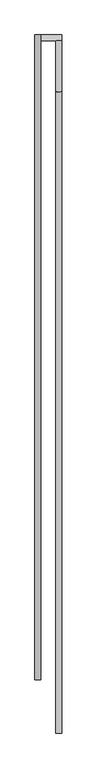
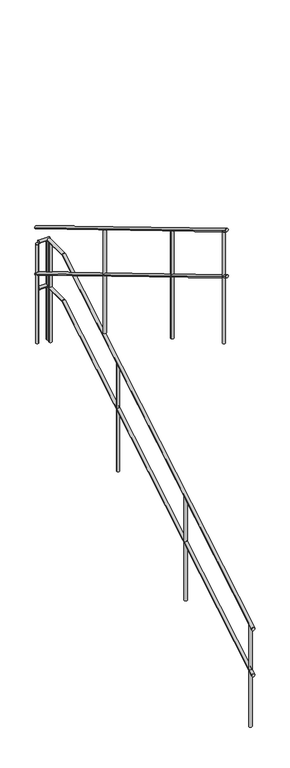
"""IFC4 building model written with IfcOpenShell, lengths in millimetres: railing geometry."""

import ifcopenshell
import ifcopenshell.guid

model = None  # the IFC model being written
_history = None  # IfcOwnerHistory: only IFC2X3 demands one
_inside = {}  # id of a spatial element -> (the spatial element, [elements in it])
_under = {}  # id of a project, library or spatial element -> (it, [spatial elements below it])
_declared = {}  # id of a project -> (the project, [libraries it declares])
_typed = {}  # id of a type object -> (the type object, [elements of that type])
_made_of = {}  # id of a material, layer set ... -> (it, [elements and type objects made of it])


def new_model(schema):
    """Start an empty IFC model of exactly this schema.

    Asked for "IFC4X3", IfcOpenShell would pick the latest addendum, in which some entities
    have other attributes; the version numbers below select the first issue.
    IFC2X3 requires an IfcOwnerHistory on every rooted entity: one is made here for all.
    """
    global model, _history
    if schema == "IFC4X3":
        model = ifcopenshell.file(schema_version=(4, 3, 0, 0))
    else:
        model = ifcopenshell.file(schema=schema)
    _inside.clear()
    _under.clear()
    _declared.clear()
    _typed.clear()
    _made_of.clear()
    _history = None
    if model.schema == "IFC2X3":
        org = make("IfcOrganization", Name="unknown")
        user = make(
            "IfcPersonAndOrganization",
            ThePerson=make("IfcPerson", FamilyName="unknown"),
            TheOrganization=org,
        )
        app = make(
            "IfcApplication",
            ApplicationDeveloper=org,
            Version="unknown",
            ApplicationFullName="unknown",
            ApplicationIdentifier="unknown",
        )
        _history = make(
            "IfcOwnerHistory",
            OwningUser=user,
            OwningApplication=app,
            ChangeAction="ADDED",
            CreationDate=0,
        )
    return model


def make(cls, **values):
    """One entity of the class cls with the attributes given. An attribute that is None is left unset."""
    return model.create_entity(
        cls, **{name: value for name, value in values.items() if value is not None}
    )


def rooted(cls, **values):
    """An entity with a GlobalId (a new one), such as an element, a storey or a relation."""
    return make(cls, GlobalId=ifcopenshell.guid.new(), OwnerHistory=_history, **values)


def si_unit(unit_type, name, prefix=None):
    """IfcSIUnit, for example si_unit("LENGTHUNIT", "METRE", prefix="MILLI")."""
    return make("IfcSIUnit", UnitType=unit_type, Prefix=prefix, Name=name)


def assignment(units):
    """IfcUnitAssignment: the units of a project."""
    return None if units is None else make("IfcUnitAssignment", Units=units)


def point(xyz):
    """IfcCartesianPoint."""
    return None if xyz is None else make("IfcCartesianPoint", Coordinates=xyz)


def direction(xyz):
    """IfcDirection."""
    return None if xyz is None else make("IfcDirection", DirectionRatios=xyz)


def frame(location, z_axis=None, x_axis=None):
    """IfcAxis2Placement3D, a coordinate frame: its origin and axes. An axis left out is left unset."""
    return make(
        "IfcAxis2Placement3D",
        Location=point(location),
        Axis=direction(z_axis),
        RefDirection=direction(x_axis),
    )


def frame_2d(location, x_axis=None):
    """IfcAxis2Placement2D, a coordinate frame in the plane: its origin and x axis."""
    return make(
        "IfcAxis2Placement2D", Location=point(location), RefDirection=direction(x_axis)
    )


def origin():
    """The frame at (0, 0, 0) with its axes left unset."""
    return frame((0.0, 0.0, 0.0))


def place(relative_to, where):
    """IfcLocalPlacement: puts the frame where relative to a parent placement (None: the world)."""
    return make(
        "IfcLocalPlacement", PlacementRelTo=relative_to, RelativePlacement=where
    )


def context(
    kind, dimensions, precision=None, world=None, true_north=None, identifier=None
):
    """IfcGeometricRepresentationContext, for example the 3D "Model" context."""
    return make(
        "IfcGeometricRepresentationContext",
        ContextIdentifier=identifier,
        ContextType=kind,
        CoordinateSpaceDimension=dimensions,
        Precision=precision,
        WorldCoordinateSystem=world,
        TrueNorth=true_north,
    )


def project(units=None, contexts=None):
    """IfcProject with its units and contexts."""
    return rooted(
        "IfcProject",
        Name="project",
        RepresentationContexts=contexts,
        UnitsInContext=assignment(units),
    )


def spatial(cls, under=None, at=None, **own):
    """A site, building, storey or space (cls), placed at a placement, below another one or the project."""
    s = rooted(cls, ObjectPlacement=at, **own)
    if under is not None:
        _under.setdefault(under.id(), (under, []))[1].append(s)
    return s


def circle_curve(where, radius):
    """IfcCircle in the frame where."""
    return make("IfcCircle", Position=where, Radius=radius)


def ellipse_curve(where, semi_axis1, semi_axis2):
    """IfcEllipse in the frame where."""
    return make(
        "IfcEllipse", Position=where, SemiAxis1=semi_axis1, SemiAxis2=semi_axis2
    )


def trimmed(basis, trim1, trim2, sense, master):
    """IfcTrimmedCurve: the piece of a basis curve between two trims."""
    return make(
        "IfcTrimmedCurve",
        BasisCurve=basis,
        Trim1=trim1,
        Trim2=trim2,
        SenseAgreement=sense,
        MasterRepresentation=master,
    )


def segment(curve, same_sense, transition):
    """IfcCompositeCurveSegment."""
    return make(
        "IfcCompositeCurveSegment",
        Transition=transition,
        SameSense=same_sense,
        ParentCurve=curve,
    )


def composite_curve(segments, self_intersect=None):
    """IfcCompositeCurve: segments joined end to end."""
    return make("IfcCompositeCurve", Segments=segments, SelfIntersect=self_intersect)


def outline(outer, holes=None, kind="AREA"):
    """IfcArbitraryClosedProfileDef: a profile drawn as a closed curve; with holes, ...WithVoids."""
    if holes is None:
        return make("IfcArbitraryClosedProfileDef", ProfileType=kind, OuterCurve=outer)
    return make(
        "IfcArbitraryProfileDefWithVoids",
        ProfileType=kind,
        OuterCurve=outer,
        InnerCurves=holes,
    )


def extrude(swept, where, along, depth):
    """IfcExtrudedAreaSolid: the profile swept, set in the frame where, extruded along a direction by depth."""
    return make(
        "IfcExtrudedAreaSolid",
        SweptArea=swept,
        Position=where,
        ExtrudedDirection=direction(along),
        Depth=depth,
    )


def shape(context_of_items, identifier, shape_type, items):
    """IfcShapeRepresentation: the items that make up one representation, for example the "Body"."""
    return make(
        "IfcShapeRepresentation",
        ContextOfItems=context_of_items,
        RepresentationIdentifier=identifier,
        RepresentationType=shape_type,
        Items=items,
    )


def source(mapping_origin, context_of_items, identifier, shape_type, items):
    """IfcRepresentationMap: a shape defined once, which mapped items show again and again."""
    return make(
        "IfcRepresentationMap",
        MappingOrigin=mapping_origin,
        MappedRepresentation=shape(context_of_items, identifier, shape_type, items),
    )


def transform(
    local_origin,
    x_axis=None,
    y_axis=None,
    z_axis=None,
    scale=None,
    scale2=None,
    scale3=None,
    uniform=True,
):
    """IfcCartesianTransformationOperator3D, or its non-uniform kind. x_axis, y_axis, z_axis: its Axis1, 2, 3."""
    if uniform:
        return make(
            "IfcCartesianTransformationOperator3D",
            Axis1=direction(x_axis),
            Axis2=direction(y_axis),
            LocalOrigin=point(local_origin),
            Scale=scale,
            Axis3=direction(z_axis),
        )
    return make(
        "IfcCartesianTransformationOperator3DnonUniform",
        Axis1=direction(x_axis),
        Axis2=direction(y_axis),
        LocalOrigin=point(local_origin),
        Scale=scale,
        Axis3=direction(z_axis),
        Scale2=scale2,
        Scale3=scale3,
    )


def mapped(mapping_source, mapping_target):
    """IfcMappedItem: shows the shape of a source again, moved by a transform."""
    return make(
        "IfcMappedItem", MappingSource=mapping_source, MappingTarget=mapping_target
    )


def made_of(thing, what):
    """Note that an element or type object is made of a material, layer set ...; save() writes the relation."""
    if what is not None:
        _made_of.setdefault(what.id(), (what, []))[1].append(thing)
    return thing


def element(
    cls,
    number,
    at=None,
    inside=None,
    cuts=None,
    type_object=None,
    material=None,
    context=None,
    identifier="Body",
    shape_type=None,
    held_by="IfcProductDefinitionShape",
    body=None,
    shapes=None,
    **own,
):
    """One element of the class cls, such as IfcWall. Its Tag is "e" and its number.

    at: its placement. inside: the storey or other place that contains it. cuts: it is an
    opening in that element (IfcRelVoidsElement). A single representation is given by context,
    identifier, shape_type and body (its items); several are given by shapes. held_by: the class
    of the entity that holds the representations. save() writes the other relations.
    """
    e = rooted(cls, Tag="e%d" % number, ObjectPlacement=at, **own)
    if body is not None:
        shapes = [shape(context, identifier, shape_type, body)]
    if shapes is not None:
        e.Representation = make(held_by, Representations=shapes)
    if inside is not None:
        _inside.setdefault(inside.id(), (inside, []))[1].append(e)
    if cuts is not None:
        rooted(
            "IfcRelVoidsElement", RelatingBuildingElement=cuts, RelatedOpeningElement=e
        )
    if type_object is not None:
        _typed.setdefault(type_object.id(), (type_object, []))[1].append(e)
    return made_of(e, material)


def aggregate(whole, parts):
    """IfcRelAggregates: a whole, such as a stair, and the parts it consists of."""
    return rooted("IfcRelAggregates", RelatingObject=whole, RelatedObjects=parts)


def save(model, path):
    """Write the relations noted so far, then the file.

    IfcRelAggregates (storeys below a building ...), IfcRelContainedInSpatialStructure (elements
    in a storey), IfcRelDefinesByType, IfcRelAssociatesMaterial and IfcRelDeclares: one each for
    every whole, place, type object, material and project.
    """
    for whole, parts in _under.values():
        aggregate(whole, parts)
    for where, things in _inside.values():
        rooted(
            "IfcRelContainedInSpatialStructure",
            RelatedElements=things,
            RelatingStructure=where,
        )
    for kind, things in _typed.values():
        rooted("IfcRelDefinesByType", RelatedObjects=things, RelatingType=kind)
    for what, things in _made_of.values():
        rooted("IfcRelAssociatesMaterial", RelatedObjects=things, RelatingMaterial=what)
    for by, libraries in _declared.values():
        rooted("IfcRelDeclares", RelatingContext=by, RelatedDefinitions=libraries)
    model.write(path)


def plane_surface(at):
    """IfcPlane: the flat surface through the origin of the frame at, square to its z axis."""
    return make("IfcPlane", Position=at)


def cylinder_surface(at, radius):
    """IfcCylindricalSurface: all points at the distance radius from the z axis of the frame at."""
    return make("IfcCylindricalSurface", Position=at, Radius=radius)


def advanced_brep(points, edges, surfaces, faces):
    """IfcAdvancedBrep: a solid bounded by faces that lie on surfaces and meet in shared edges.

    An edge is (start, end): straight between two places in points (the first is 0);
    or (start, end, curve); or (start, end, curve, False) where it runs against its curve.
    A face is (place in surfaces, loops), or (place, loops, False) where it looks against
    its surface's normal. A loop lists edges by number (the first is 1), with a minus sign
    where the edge is run from its end to its start. The first loop is the outer one.
    """
    corners = [point(p) for p in points]
    vertices = [make("IfcVertexPoint", VertexGeometry=c) for c in corners]
    made = []
    for start, end, *more in edges:
        made.append(
            make(
                "IfcEdgeCurve",
                EdgeStart=vertices[start],
                EdgeEnd=vertices[end],
                EdgeGeometry=more[0] if more else make("IfcPolyline", Points=[corners[start], corners[end]]),
                SameSense=more[1] if len(more) > 1 else True,
            )
        )
    hull = []
    for where, loops, *sense in faces:
        bounds = []
        for j, loop in enumerate(loops):
            ring = [make("IfcOrientedEdge", EdgeElement=made[abs(k) - 1], Orientation=k > 0) for k in loop]
            bounds.append(
                make(
                    "IfcFaceOuterBound" if j == 0 else "IfcFaceBound",
                    Bound=make("IfcEdgeLoop", EdgeList=ring),
                    Orientation=True,
                )
            )
        hull.append(make("IfcAdvancedFace", Bounds=bounds, FaceSurface=surfaces[where], SameSense=sense[0] if sense else True))
    return make("IfcAdvancedBrep", Outer=make("IfcClosedShell", CfsFaces=hull))


def railing_6fbbbaa8(model_context):
    return source(origin(), model_context, "Body", "SolidModel", [
        advanced_brep(
        [(11545.1052251, 14699.5208589, 749.8338893), (11515.1052251, 14699.5208589, 749.8338893), (11545.1052251, 18329.5208589, 2760.0), (11515.1052251, 18329.5208589, 2760.0), (11545.1052251, 18063.6609247, 2760.0), (11515.1052251, 18063.6609247, 2760.0)],
        [
            (0, 1, ellipse_curve(frame((11530.1052251, 14699.5208589, 749.8338893), z_axis=(0.0, -1.0, 0.0), x_axis=(0.0, 0.0, -1.0)), 17.4738031, 15.0)),
            (1, 0, ellipse_curve(frame((11530.1052251, 14699.5208589, 749.8338893), z_axis=(0.0, -1.0, 0.0), x_axis=(0.0, 0.0, -1.0)), 17.4738031, 15.0)),
            (2, 3, circle_curve(frame((11530.1052251, 18329.5208589, 2760.0), z_axis=(0.0, 1.0, 0.0), x_axis=(-1.0, 0.0, 0.0)), 15.0)),
            (3, 2, circle_curve(frame((11530.1052251, 18329.5208589, 2760.0), z_axis=(0.0, 1.0, 0.0), x_axis=(-1.0, 0.0, 0.0)), 15.0)),
            (0, 4),
            (4, 5, ellipse_curve(frame((11530.1052251, 18063.6609247, 2760.0), z_axis=(0.0, -0.9639574411334471, -0.26605648213012423), x_axis=(0.0, 0.2660564821301243, -0.9639574411334468)), 15.560853, 15.0)),
            (5, 1),
            (5, 4, ellipse_curve(frame((11530.1052251, 18063.6609247, 2760.0), z_axis=(0.0, -0.9639574411334471, -0.26605648213012423), x_axis=(0.0, 0.2660564821301243, -0.9639574411334468)), 15.560853, 15.0)),
            (4, 2),
            (3, 5),
        ],
        [
            plane_surface(frame((11530.1052251, 14699.5208589, 767.3076923), z_axis=(0.0, -1.0, 0.0), x_axis=(0.0, 0.0, 1.0))),
            plane_surface(frame((11530.1052251, 18329.5208589, 2775.0), z_axis=(0.0, 1.0, 0.0), x_axis=(0.0, 0.0, 1.0))),
            cylinder_surface(frame((11530.1052251, 14707.2148727, 754.4312739), z_axis=(0.0, -0.8584278966330859, -0.5129342514222422), x_axis=(-1.0, 0.0, 0.0)), 15.0),
            cylinder_surface(frame((11530.1052251, 18059.5208589, 2760.0), z_axis=(0.0, -1.0, 0.0), x_axis=(-1.0, 0.0, 0.0)), 15.0),
        ],
        [
            (0, [[1, 2]]),
            (1, [[3, 4]]),
            (2, [[-1, 5, 6, 7]]),
            (2, [[-2, -7, 8, -5]]),
            (3, [[-6, 9, -4, 10]]),
            (3, [[-8, -10, -3, -9]]),
        ],
    ),
        advanced_brep(
        [(11545.1052251, 18359.5208589, 2760.0), (11545.1052251, 18329.5208589, 2760.0), (11435.1052251, 18359.5208589, 2760.0), (11435.1052251, 18329.5208589, 2760.0)],
        [
            (0, 1, circle_curve(frame((11545.1052251, 18344.5208589, 2760.0), z_axis=(1.0, 0.0, 0.0), x_axis=(0.0, -1.0, 0.0)), 15.0)),
            (1, 0, circle_curve(frame((11545.1052251, 18344.5208589, 2760.0), z_axis=(1.0, 0.0, 0.0), x_axis=(0.0, -1.0, 0.0)), 15.0)),
            (2, 3, circle_curve(frame((11435.1052251, 18344.5208589, 2760.0), z_axis=(-1.0, 0.0, 0.0), x_axis=(0.0, -1.0, 0.0)), 15.0)),
            (3, 2, circle_curve(frame((11435.1052251, 18344.5208589, 2760.0), z_axis=(-1.0, 0.0, 0.0), x_axis=(0.0, -1.0, 0.0)), 15.0)),
            (0, 2),
            (3, 1),
        ],
        [
            plane_surface(frame((11545.1052251, 18344.5208589, 2775.0), z_axis=(1.0, 0.0, 0.0), x_axis=(0.0, -1.0, 0.0))),
            plane_surface(frame((11435.1052251, 18344.5208589, 2775.0), z_axis=(-1.0, 0.0, 0.0), x_axis=(0.0, -1.0, 0.0))),
            cylinder_surface(frame((11545.1052251, 18344.5208589, 2760.0), z_axis=(1.0, 0.0, 0.0), x_axis=(0.0, -1.0, 0.0)), 15.0),
        ],
        [
            (0, [[1, 2]]),
            (1, [[3, 4]]),
            (2, [[-1, 5, -4, 6]]),
            (2, [[-2, -6, -3, -5]]),
        ],
    ),
        advanced_brep(
        [(11405.1052251, 18359.5208589, 2912.8833398), (11435.1052251, 18359.5208589, 2912.8833398), (11405.1052251, 14979.5208589, 4932.5261969), (11435.1052251, 14979.5208589, 4932.5261969)],
        [
            (0, 1, ellipse_curve(frame((11420.1052251, 18359.5208589, 2912.8833398), z_axis=(0.0, 1.0, 0.0), x_axis=(0.0, 0.0, -1.0)), 17.4738031, 15.0)),
            (1, 0, ellipse_curve(frame((11420.1052251, 18359.5208589, 2912.8833398), z_axis=(0.0, 1.0, 0.0), x_axis=(0.0, 0.0, -1.0)), 17.4738031, 15.0)),
            (2, 3, ellipse_curve(frame((11420.1052251, 14979.5208589, 4932.5261969), z_axis=(0.0, -1.0, 0.0), x_axis=(0.0, 0.0, -1.0)), 17.4738031, 15.0)),
            (3, 2, ellipse_curve(frame((11420.1052251, 14979.5208589, 4932.5261969), z_axis=(0.0, -1.0, 0.0), x_axis=(0.0, 0.0, -1.0)), 17.4738031, 15.0)),
            (0, 2),
            (3, 1),
        ],
        [
            plane_surface(frame((11420.1052251, 18359.5208589, 2930.3571429), z_axis=(0.0, 1.0, 0.0), x_axis=(0.0, 0.0, -1.0))),
            plane_surface(frame((11420.1052251, 14979.5208589, 4950.0), z_axis=(0.0, -1.0, 0.0), x_axis=(0.0, 0.0, -1.0))),
            cylinder_surface(frame((11420.1052251, 18351.8268451, 2917.4807244), z_axis=(0.0, 0.8584278966330859, -0.5129342514222421), x_axis=(1.0, 0.0, 0.0)), 15.0),
        ],
        [
            (0, [[1, 2]]),
            (1, [[3, 4]]),
            (2, [[-1, 5, -4, 6]]),
            (2, [[-2, -6, -3, -5]]),
        ],
    ),
        advanced_brep(
        [(11545.1052251, 14699.5208589, 1249.8338893), (11515.1052251, 14699.5208589, 1249.8338893), (11545.1052251, 18063.6609247, 3260.0), (11515.1052251, 18063.6609247, 3260.0), (11545.1052251, 18329.5208589, 3260.0), (11515.1052251, 18329.5208589, 3260.0)],
        [
            (0, 1, ellipse_curve(frame((11530.1052251, 14699.5208589, 1249.8338893), z_axis=(0.0, -1.0, 0.0), x_axis=(0.0, 0.0, -1.0)), 17.4738031, 15.0)),
            (1, 0, ellipse_curve(frame((11530.1052251, 14699.5208589, 1249.8338893), z_axis=(0.0, -1.0, 0.0), x_axis=(0.0, 0.0, -1.0)), 17.4738031, 15.0)),
            (0, 2),
            (2, 3, ellipse_curve(frame((11530.1052251, 18063.6609247, 3260.0), z_axis=(0.0, -0.9639574411334471, -0.26605648213012423), x_axis=(0.0, 0.2660564821301243, -0.9639574411334468)), 15.560853, 15.0)),
            (3, 1),
            (3, 2, ellipse_curve(frame((11530.1052251, 18063.6609247, 3260.0), z_axis=(0.0, -0.9639574411334471, -0.26605648213012423), x_axis=(0.0, 0.2660564821301243, -0.9639574411334468)), 15.560853, 15.0)),
            (4, 5, circle_curve(frame((11530.1052251, 18329.5208589, 3260.0), z_axis=(0.0, 1.0, 0.0), x_axis=(-1.0, 0.0, 0.0)), 15.0)),
            (5, 4, circle_curve(frame((11530.1052251, 18329.5208589, 3260.0), z_axis=(0.0, 1.0, 0.0), x_axis=(-1.0, 0.0, 0.0)), 15.0)),
            (2, 4),
            (5, 3),
        ],
        [
            plane_surface(frame((11530.1052251, 14699.5208589, 1267.3076923), z_axis=(0.0, -1.0, 0.0), x_axis=(0.0, 0.0, 1.0))),
            cylinder_surface(frame((11530.1052251, 14707.2148727, 1254.4312739), z_axis=(0.0, -0.8584278966330859, -0.5129342514222422), x_axis=(-1.0, 0.0, 0.0)), 15.0),
            plane_surface(frame((11530.1052251, 18329.5208589, 3275.0), z_axis=(0.0, 1.0, 0.0), x_axis=(0.0, 0.0, 1.0))),
            cylinder_surface(frame((11530.1052251, 18059.5208589, 3260.0), z_axis=(0.0, -1.0, 0.0), x_axis=(-1.0, 0.0, 0.0)), 15.0),
        ],
        [
            (0, [[1, 2]]),
            (1, [[-1, 3, 4, 5]]),
            (1, [[-2, -5, 6, -3]]),
            (2, [[7, 8]]),
            (3, [[-4, 9, -8, 10]]),
            (3, [[-6, -10, -7, -9]]),
        ],
    ),
        advanced_brep(
        [(11545.1052251, 18359.5208589, 3260.0), (11545.1052251, 18329.5208589, 3260.0), (11435.1052251, 18359.5208589, 3260.0), (11435.1052251, 18329.5208589, 3260.0)],
        [
            (0, 1, circle_curve(frame((11545.1052251, 18344.5208589, 3260.0), z_axis=(1.0, 0.0, 0.0), x_axis=(0.0, -1.0, 0.0)), 15.0)),
            (1, 0, circle_curve(frame((11545.1052251, 18344.5208589, 3260.0), z_axis=(1.0, 0.0, 0.0), x_axis=(0.0, -1.0, 0.0)), 15.0)),
            (2, 3, circle_curve(frame((11435.1052251, 18344.5208589, 3260.0), z_axis=(-1.0, 0.0, 0.0), x_axis=(0.0, -1.0, 0.0)), 15.0)),
            (3, 2, circle_curve(frame((11435.1052251, 18344.5208589, 3260.0), z_axis=(-1.0, 0.0, 0.0), x_axis=(0.0, -1.0, 0.0)), 15.0)),
            (0, 2),
            (3, 1),
        ],
        [
            plane_surface(frame((11545.1052251, 18344.5208589, 3275.0), z_axis=(1.0, 0.0, 0.0), x_axis=(0.0, -1.0, 0.0))),
            plane_surface(frame((11435.1052251, 18344.5208589, 3275.0), z_axis=(-1.0, 0.0, 0.0), x_axis=(0.0, -1.0, 0.0))),
            cylinder_surface(frame((11545.1052251, 18344.5208589, 3260.0), z_axis=(1.0, 0.0, 0.0), x_axis=(0.0, -1.0, 0.0)), 15.0),
        ],
        [
            (0, [[1, 2]]),
            (1, [[3, 4]]),
            (2, [[-1, 5, -4, 6]]),
            (2, [[-2, -6, -3, -5]]),
        ],
    ),
        advanced_brep(
        [(11405.1052251, 18359.5208589, 3412.8833398), (11435.1052251, 18359.5208589, 3412.8833398), (11405.1052251, 14979.5208589, 5432.5261969), (11435.1052251, 14979.5208589, 5432.5261969)],
        [
            (0, 1, ellipse_curve(frame((11420.1052251, 18359.5208589, 3412.8833398), z_axis=(0.0, 1.0, 0.0), x_axis=(0.0, 0.0, -1.0)), 17.4738031, 15.0)),
            (1, 0, ellipse_curve(frame((11420.1052251, 18359.5208589, 3412.8833398), z_axis=(0.0, 1.0, 0.0), x_axis=(0.0, 0.0, -1.0)), 17.4738031, 15.0)),
            (2, 3, ellipse_curve(frame((11420.1052251, 14979.5208589, 5432.5261969), z_axis=(0.0, -1.0, 0.0), x_axis=(0.0, 0.0, -1.0)), 17.4738031, 15.0)),
            (3, 2, ellipse_curve(frame((11420.1052251, 14979.5208589, 5432.5261969), z_axis=(0.0, -1.0, 0.0), x_axis=(0.0, 0.0, -1.0)), 17.4738031, 15.0)),
            (0, 2),
            (3, 1),
        ],
        [
            plane_surface(frame((11420.1052251, 18359.5208589, 3430.3571429), z_axis=(0.0, 1.0, 0.0), x_axis=(0.0, 0.0, -1.0))),
            plane_surface(frame((11420.1052251, 14979.5208589, 5450.0), z_axis=(0.0, -1.0, 0.0), x_axis=(0.0, 0.0, -1.0))),
            cylinder_surface(frame((11420.1052251, 18351.8268451, 3417.4807244), z_axis=(0.0, 0.8584278966330859, -0.5129342514222421), x_axis=(1.0, 0.0, 0.0)), 15.0),
        ],
        [
            (0, [[1, 2]]),
            (1, [[3, 4]]),
            (2, [[-1, 5, -4, 6]]),
            (2, [[-2, -6, -3, -5]]),
        ],
    ),
        extrude(outline(composite_curve([segment(trimmed(circle_curve(frame_2d((11420.1052251, 15944.5208589)), 15.0), [point((11435.1052251, 15944.5208589))], [point((11405.1052251, 15944.5208589))], False, "CARTESIAN"), True, "CONTINUOUS"), segment(trimmed(circle_curve(frame_2d((11420.1052251, 15944.5208589)), 15.0), [point((11405.1052251, 15944.5208589))], [point((11435.1052251, 15944.5208589))], False, "CARTESIAN"), True, "CONTINUOUS")], self_intersect=False)), frame((0.0, 0.0, 3680.7692308), z_axis=(0.0, 0.0, 1.0), x_axis=(1.0, 0.0, 0.0)), (0.0, 0.0, 1.0), 1162.6167582),
        extrude(outline(composite_curve([segment(trimmed(circle_curve(frame_2d((11420.1052251, 17144.5208589)), 15.0), [point((11435.1052251, 17144.5208589))], [point((11405.1052251, 17144.5208589))], False, "CARTESIAN"), True, "CONTINUOUS"), segment(trimmed(circle_curve(frame_2d((11420.1052251, 17144.5208589)), 15.0), [point((11405.1052251, 17144.5208589))], [point((11435.1052251, 17144.5208589))], False, "CARTESIAN"), True, "CONTINUOUS")], self_intersect=False)), frame((0.0, 0.0, 3011.5384615), z_axis=(0.0, 0.0, 1.0), x_axis=(1.0, 0.0, 0.0)), (0.0, 0.0, 1.0), 1114.8145604),
        extrude(outline(composite_curve([segment(trimmed(circle_curve(frame_2d((11530.1052251, 18299.5208589)), 15.0), [point((11515.1052251, 18299.5208589))], [point((11545.1052251, 18299.5208589))], False, "CARTESIAN"), True, "CONTINUOUS"), segment(trimmed(circle_curve(frame_2d((11530.1052251, 18299.5208589)), 15.0), [point((11545.1052251, 18299.5208589))], [point((11515.1052251, 18299.5208589))], False, "CARTESIAN"), True, "CONTINUOUS")], self_intersect=False)), frame((0.0, 0.0, 2175.0), z_axis=(0.0, 0.0, 1.0), x_axis=(1.0, 0.0, 0.0)), (0.0, 0.0, 1.0), 1070.0),
        extrude(outline(composite_curve([segment(trimmed(circle_curve(frame_2d((11530.1052251, 17099.5208589)), 15.0), [point((11515.1052251, 17099.5208589))], [point((11545.1052251, 17099.5208589))], False, "CARTESIAN"), True, "CONTINUOUS"), segment(trimmed(circle_curve(frame_2d((11530.1052251, 17099.5208589)), 15.0), [point((11545.1052251, 17099.5208589))], [point((11515.1052251, 17099.5208589))], False, "CARTESIAN"), True, "CONTINUOUS")], self_intersect=False)), frame((0.0, 0.0, 1505.7692308), z_axis=(0.0, 0.0, 1.0), x_axis=(1.0, 0.0, 0.0)), (0.0, 0.0, 1.0), 1165.6043956),
        extrude(outline(composite_curve([segment(trimmed(circle_curve(frame_2d((11530.1052251, 15899.5208589)), 15.0), [point((11515.1052251, 15899.5208589))], [point((11545.1052251, 15899.5208589))], False, "CARTESIAN"), True, "CONTINUOUS"), segment(trimmed(circle_curve(frame_2d((11530.1052251, 15899.5208589)), 15.0), [point((11545.1052251, 15899.5208589))], [point((11515.1052251, 15899.5208589))], False, "CARTESIAN"), True, "CONTINUOUS")], self_intersect=False)), frame((0.0, 0.0, 836.5384615), z_axis=(0.0, 0.0, 1.0), x_axis=(1.0, 0.0, 0.0)), (0.0, 0.0, 1.0), 1117.8021978),
        extrude(outline(composite_curve([segment(trimmed(circle_curve(frame_2d((11420.1052251, 18344.5208589)), 15.0), [point((11420.1052251, 18329.5208589))], [point((11420.1052251, 18359.5208589))], False, "CARTESIAN"), True, "CONTINUOUS"), segment(trimmed(circle_curve(frame_2d((11420.1052251, 18344.5208589)), 15.0), [point((11420.1052251, 18359.5208589))], [point((11420.1052251, 18329.5208589))], False, "CARTESIAN"), True, "CONTINUOUS")], self_intersect=False)), frame((0.0, 0.0, 2175.0), z_axis=(0.0, 0.0, 1.0), x_axis=(1.0, 0.0, 0.0)), (0.0, 0.0, 1.0), 1070.0),
        extrude(outline(composite_curve([segment(trimmed(circle_curve(frame_2d((11530.1052251, 18344.5208589)), 15.0), [point((11515.1052251, 18344.5208589))], [point((11545.1052251, 18344.5208589))], False, "CARTESIAN"), True, "CONTINUOUS"), segment(trimmed(circle_curve(frame_2d((11530.1052251, 18344.5208589)), 15.0), [point((11545.1052251, 18344.5208589))], [point((11515.1052251, 18344.5208589))], False, "CARTESIAN"), True, "CONTINUOUS")], self_intersect=False)), frame((0.0, 0.0, 2175.0), z_axis=(0.0, 0.0, 1.0), x_axis=(1.0, 0.0, 0.0)), (0.0, 0.0, 1.0), 1070.0),
        extrude(outline(composite_curve([segment(trimmed(circle_curve(frame_2d((11420.1052251, 15029.5208589)), 15.0), [point((11435.1052251, 15029.5208589))], [point((11405.1052251, 15029.5208589))], False, "CARTESIAN"), True, "CONTINUOUS"), segment(trimmed(circle_curve(frame_2d((11420.1052251, 15029.5208589)), 15.0), [point((11405.1052251, 15029.5208589))], [point((11435.1052251, 15029.5208589))], False, "CARTESIAN"), True, "CONTINUOUS")], self_intersect=False)), frame((0.0, 0.0, 4182.6923077), z_axis=(0.0, 0.0, 1.0), x_axis=(1.0, 0.0, 0.0)), (0.0, 0.0, 1.0), 1207.4313187),
        extrude(outline(composite_curve([segment(trimmed(circle_curve(frame_2d((11530.1052251, 14749.5208589)), 15.0), [point((11515.1052251, 14749.5208589))], [point((11545.1052251, 14749.5208589))], False, "CARTESIAN"), True, "CONTINUOUS"), segment(trimmed(circle_curve(frame_2d((11530.1052251, 14749.5208589)), 15.0), [point((11545.1052251, 14749.5208589))], [point((11515.1052251, 14749.5208589))], False, "CARTESIAN"), True, "CONTINUOUS")], self_intersect=False)), frame((0.0, 0.0, 167.3076923), z_axis=(0.0, 0.0, 1.0), x_axis=(1.0, 0.0, 0.0)), (0.0, 0.0, 1.0), 1099.8763736),
    ])


if __name__ == "__main__":
    model = new_model("IFC4")
    model_context = context("Model", 3, world=origin())
    ifc_project = project(units=[si_unit("LENGTHUNIT", "METRE", prefix="MILLI")], contexts=[model_context])
    site = spatial("IfcSite", under=ifc_project)
    building = spatial("IfcBuilding", under=site)
    placement = place(None, origin())
    railing_shape = railing_6fbbbaa8(model_context)
    element("IfcRailing", 1, at=placement, inside=building, context=model_context, shape_type="MappedRepresentation", body=[
        mapped(railing_shape, transform((0.0, 0.0, 0.0), x_axis=(1.0, 0.0, 0.0), y_axis=(0.0, 1.0, 0.0), z_axis=(0.0, 0.0, 1.0))),
    ])
    save(model, "model.ifc")
